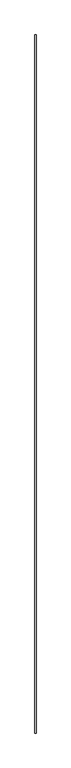
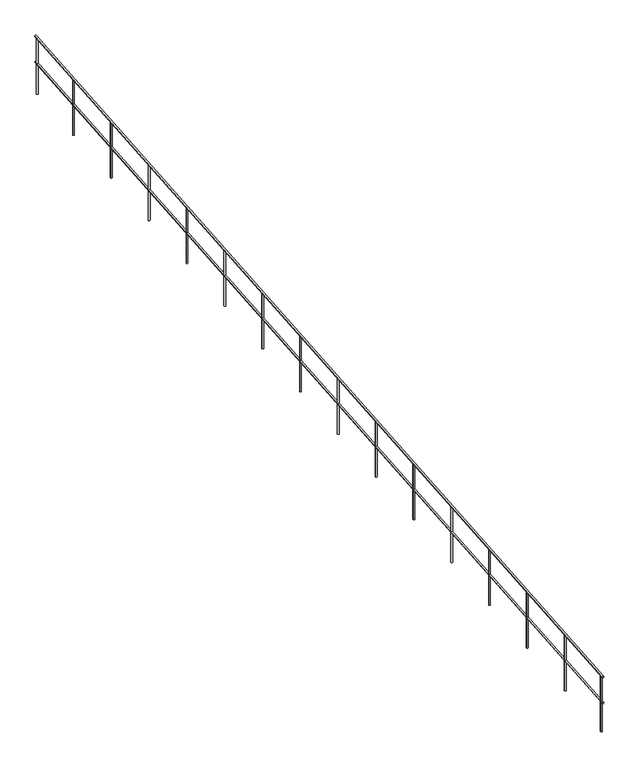
"""IFC4 building model written with IfcOpenShell, lengths in millimetres: railing geometry."""

from ifc_helpers import new_model, si_unit, frame, origin, place, context, project, spatial, ellipse_curve, source, transform, mapped, element, save
from ifc_brep_helpers import plane_surface, cylinder_surface, advanced_brep


def railing_739abddc(model_context):
    return source(origin(), model_context, "Body", "AdvancedBrep", [
        advanced_brep(
        [(-4051.0, 39498.9598199, -615.0519932), (-4081.0, 39498.9598199, -615.0519932), (-4051.0, 57498.9598198, 884.9480068), (-4081.0, 57498.9598198, 884.9480068)],
        [
            (0, 1, ellipse_curve(frame((-4066.0, 39498.9598199, -615.0519932), z_axis=(0.0, -1.0, 0.0), x_axis=(0.0, 0.0, -0.9999999999999999)), 15.0519932, 15.0)),
            (1, 0, ellipse_curve(frame((-4066.0, 39498.9598199, -615.0519932), z_axis=(0.0, -1.0, 0.0), x_axis=(0.0, 0.0, -0.9999999999999999)), 15.0519932, 15.0)),
            (2, 3, ellipse_curve(frame((-4066.0, 57498.9598198, 884.9480068), z_axis=(0.0, 1.0, 0.0), x_axis=(0.0, 0.0, -0.9999999999999999)), 15.0519932, 15.0)),
            (3, 2, ellipse_curve(frame((-4066.0, 57498.9598198, 884.9480068), z_axis=(0.0, 1.0, 0.0), x_axis=(0.0, 0.0, -0.9999999999999999)), 15.0519932, 15.0)),
            (0, 2),
            (3, 1),
        ],
        [
            plane_surface(frame((-4066.0, 39498.9598199, -600.0), z_axis=(0.0, -1.0, 0.0), x_axis=(0.0, 0.0, 1.0))),
            plane_surface(frame((-4066.0, 57498.9598198, 900.0), z_axis=(0.0, 1.0, 0.0), x_axis=(0.0, 0.0, 1.0))),
            cylinder_surface(frame((-4066.0, 39500.2055021, -614.9481864), z_axis=(0.0, -0.9965457582448797, -0.08304547985373997), x_axis=(-1.0, 0.0, 0.0)), 15.0),
        ],
        [
            (0, [[1, 2]]),
            (1, [[3, 4]]),
            (2, [[-1, 5, -4, 6]]),
            (2, [[-2, -6, -3, -5]]),
        ],
    ),
        advanced_brep(
        [(-4051.0, 39498.9598199, -115.0519932), (-4081.0, 39498.9598199, -115.0519932), (-4051.0, 57498.9598198, 1384.9480068), (-4081.0, 57498.9598198, 1384.9480068)],
        [
            (0, 1, ellipse_curve(frame((-4066.0, 39498.9598199, -115.0519932), z_axis=(0.0, -1.0, 0.0), x_axis=(0.0, 0.0, -0.9999999999999999)), 15.0519932, 15.0)),
            (1, 0, ellipse_curve(frame((-4066.0, 39498.9598199, -115.0519932), z_axis=(0.0, -1.0, 0.0), x_axis=(0.0, 0.0, -0.9999999999999999)), 15.0519932, 15.0)),
            (2, 3, ellipse_curve(frame((-4066.0, 57498.9598198, 1384.9480068), z_axis=(0.0, 1.0, 0.0), x_axis=(0.0, 0.0, -0.9999999999999999)), 15.0519932, 15.0)),
            (3, 2, ellipse_curve(frame((-4066.0, 57498.9598198, 1384.9480068), z_axis=(0.0, 1.0, 0.0), x_axis=(0.0, 0.0, -0.9999999999999999)), 15.0519932, 15.0)),
            (0, 2),
            (3, 1),
        ],
        [
            plane_surface(frame((-4066.0, 39498.9598199, -100.0), z_axis=(0.0, -1.0, 0.0), x_axis=(0.0, 0.0, 1.0))),
            plane_surface(frame((-4066.0, 57498.9598198, 1400.0), z_axis=(0.0, 1.0, 0.0), x_axis=(0.0, 0.0, 1.0))),
            cylinder_surface(frame((-4066.0, 39500.2055021, -114.9481864), z_axis=(0.0, -0.9965457582448797, -0.08304547985373997), x_axis=(-1.0, 0.0, 0.0)), 15.0),
        ],
        [
            (0, [[1, 2]]),
            (1, [[3, 4]]),
            (2, [[-1, 5, -4, 6]]),
            (2, [[-2, -6, -3, -5]]),
        ],
    ),
        advanced_brep(
        [(-4081.0, 56298.9598199, 1269.8960136), (-4051.0, 56298.9598199, 1269.8960136), (-4051.0, 56298.9598199, 200.0), (-4081.0, 56298.9598199, 200.0)],
        [
            (0, 1, ellipse_curve(frame((-4066.0, 56298.9598199, 1269.8960136), z_axis=(0.0, 0.083045479853741, -0.9965457582448796), x_axis=(0.0, 0.9965457582448797, 0.08304547985374044)), 15.0519932, 15.0)),
            (1, 2),
            (2, 3, ellipse_curve(frame((-4066.0, 56298.9598199, 200.0), z_axis=(0.0, -0.08304547985373996, 0.9965457582448797), x_axis=(0.0, 0.9965457582448798, 0.08304547985373881)), 15.0519932, 15.0)),
            (3, 0),
            (3, 2, ellipse_curve(frame((-4066.0, 56298.9598199, 200.0), z_axis=(0.0, -0.08304547985373996, 0.9965457582448797), x_axis=(0.0, 0.9965457582448798, 0.08304547985373881)), 15.0519932, 15.0)),
            (1, 0, ellipse_curve(frame((-4066.0, 56298.9598199, 1269.8960136), z_axis=(0.0, 0.083045479853741, -0.9965457582448796), x_axis=(0.0, 0.9965457582448797, 0.08304547985374044)), 15.0519932, 15.0)),
        ],
        [
            cylinder_surface(frame((-4066.0, 56298.9598199, 100.0), z_axis=(0.0, 0.0, 1.0), x_axis=(1.0, 0.0, 0.0)), 15.0),
            plane_surface(frame((-4041.0, 56323.9598199, 1271.9793469), z_axis=(0.0, -0.083045479853741, 0.9965457582448796), x_axis=(-1.0, 0.0, 0.0))),
            plane_surface(frame((-4041.0, 56273.9598199, 197.9166667), z_axis=(0.0, 0.08304547985373996, -0.9965457582448797), x_axis=(-1.0, 0.0, 0.0))),
        ],
        [
            (0, [[1, 2, 3, 4]]),
            (0, [[5, -2, 6, -4]]),
            (1, [[-6, -1]]),
            (2, [[-5, -3]]),
        ],
    ),
        advanced_brep(
        [(-4081.0, 55098.9598199, 1169.8960136), (-4051.0, 55098.9598199, 1169.8960136), (-4051.0, 55098.9598199, 100.0), (-4081.0, 55098.9598199, 100.0)],
        [
            (0, 1, ellipse_curve(frame((-4066.0, 55098.9598199, 1169.8960136), z_axis=(0.0, 0.083045479853741, -0.9965457582448796), x_axis=(0.0, 0.9965457582448797, 0.08304547985374044)), 15.0519932, 15.0)),
            (1, 2),
            (2, 3, ellipse_curve(frame((-4066.0, 55098.9598199, 100.0), z_axis=(0.0, -0.08304547985373996, 0.9965457582448797), x_axis=(0.0, 0.9965457582448798, 0.08304547985373881)), 15.0519932, 15.0)),
            (3, 0),
            (3, 2, ellipse_curve(frame((-4066.0, 55098.9598199, 100.0), z_axis=(0.0, -0.08304547985373996, 0.9965457582448797), x_axis=(0.0, 0.9965457582448798, 0.08304547985373881)), 15.0519932, 15.0)),
            (1, 0, ellipse_curve(frame((-4066.0, 55098.9598199, 1169.8960136), z_axis=(0.0, 0.083045479853741, -0.9965457582448796), x_axis=(0.0, 0.9965457582448797, 0.08304547985374044)), 15.0519932, 15.0)),
        ],
        [
            cylinder_surface(frame((-4066.0, 55098.9598199, 0.0), z_axis=(0.0, 0.0, 1.0), x_axis=(1.0, 0.0, 0.0)), 15.0),
            plane_surface(frame((-4041.0, 55123.9598199, 1171.9793469), z_axis=(0.0, -0.083045479853741, 0.9965457582448796), x_axis=(-1.0, 0.0, 0.0))),
            plane_surface(frame((-4041.0, 55073.9598199, 97.9166667), z_axis=(0.0, 0.08304547985373996, -0.9965457582448797), x_axis=(-1.0, 0.0, 0.0))),
        ],
        [
            (0, [[1, 2, 3, 4]]),
            (0, [[5, -2, 6, -4]]),
            (1, [[-6, -1]]),
            (2, [[-5, -3]]),
        ],
    ),
        advanced_brep(
        [(-4081.0, 53898.9598199, 1069.8960136), (-4051.0, 53898.9598199, 1069.8960136), (-4051.0, 53898.9598199, 0.0), (-4081.0, 53898.9598199, 0.0)],
        [
            (0, 1, ellipse_curve(frame((-4066.0, 53898.9598199, 1069.8960136), z_axis=(0.0, 0.083045479853741, -0.9965457582448796), x_axis=(0.0, 0.9965457582448797, 0.08304547985374044)), 15.0519932, 15.0)),
            (1, 2),
            (2, 3, ellipse_curve(frame((-4066.0, 53898.9598199, 0.0), z_axis=(0.0, -0.08304547985373996, 0.9965457582448797), x_axis=(0.0, 0.9965457582448798, 0.08304547985373881)), 15.0519932, 15.0)),
            (3, 0),
            (3, 2, ellipse_curve(frame((-4066.0, 53898.9598199, 0.0), z_axis=(0.0, -0.08304547985373996, 0.9965457582448797), x_axis=(0.0, 0.9965457582448798, 0.08304547985373881)), 15.0519932, 15.0)),
            (1, 0, ellipse_curve(frame((-4066.0, 53898.9598199, 1069.8960136), z_axis=(0.0, 0.083045479853741, -0.9965457582448796), x_axis=(0.0, 0.9965457582448797, 0.08304547985374044)), 15.0519932, 15.0)),
        ],
        [
            cylinder_surface(frame((-4066.0, 53898.9598199, -100.0), z_axis=(0.0, 0.0, 1.0), x_axis=(1.0, 0.0, 0.0)), 15.0),
            plane_surface(frame((-4041.0, 53923.9598199, 1071.9793469), z_axis=(0.0, -0.083045479853741, 0.9965457582448796), x_axis=(-1.0, 0.0, 0.0))),
            plane_surface(frame((-4041.0, 53873.9598199, -2.0833333), z_axis=(0.0, 0.08304547985373996, -0.9965457582448797), x_axis=(-1.0, 0.0, 0.0))),
        ],
        [
            (0, [[1, 2, 3, 4]]),
            (0, [[5, -2, 6, -4]]),
            (1, [[-6, -1]]),
            (2, [[-5, -3]]),
        ],
    ),
        advanced_brep(
        [(-4081.0, 52698.9598199, 969.8960136), (-4051.0, 52698.9598199, 969.8960136), (-4051.0, 52698.9598199, -100.0), (-4081.0, 52698.9598199, -100.0)],
        [
            (0, 1, ellipse_curve(frame((-4066.0, 52698.9598199, 969.8960136), z_axis=(0.0, 0.083045479853741, -0.9965457582448796), x_axis=(0.0, 0.9965457582448797, 0.08304547985374044)), 15.0519932, 15.0)),
            (1, 2),
            (2, 3, ellipse_curve(frame((-4066.0, 52698.9598199, -100.0), z_axis=(0.0, -0.08304547985373996, 0.9965457582448797), x_axis=(0.0, 0.9965457582448798, 0.08304547985373881)), 15.0519932, 15.0)),
            (3, 0),
            (3, 2, ellipse_curve(frame((-4066.0, 52698.9598199, -100.0), z_axis=(0.0, -0.08304547985373996, 0.9965457582448797), x_axis=(0.0, 0.9965457582448798, 0.08304547985373881)), 15.0519932, 15.0)),
            (1, 0, ellipse_curve(frame((-4066.0, 52698.9598199, 969.8960136), z_axis=(0.0, 0.083045479853741, -0.9965457582448796), x_axis=(0.0, 0.9965457582448797, 0.08304547985374044)), 15.0519932, 15.0)),
        ],
        [
            cylinder_surface(frame((-4066.0, 52698.9598199, -200.0), z_axis=(0.0, 0.0, 1.0), x_axis=(1.0, 0.0, 0.0)), 15.0),
            plane_surface(frame((-4041.0, 52723.9598199, 971.9793469), z_axis=(0.0, -0.083045479853741, 0.9965457582448796), x_axis=(-1.0, 0.0, 0.0))),
            plane_surface(frame((-4041.0, 52673.9598199, -102.0833333), z_axis=(0.0, 0.08304547985373996, -0.9965457582448797), x_axis=(-1.0, 0.0, 0.0))),
        ],
        [
            (0, [[1, 2, 3, 4]]),
            (0, [[5, -2, 6, -4]]),
            (1, [[-6, -1]]),
            (2, [[-5, -3]]),
        ],
    ),
        advanced_brep(
        [(-4081.0, 51498.9598199, 869.8960136), (-4051.0, 51498.9598199, 869.8960136), (-4051.0, 51498.9598199, -200.0), (-4081.0, 51498.9598199, -200.0)],
        [
            (0, 1, ellipse_curve(frame((-4066.0, 51498.9598199, 869.8960136), z_axis=(0.0, 0.083045479853741, -0.9965457582448796), x_axis=(0.0, 0.9965457582448797, 0.08304547985374044)), 15.0519932, 15.0)),
            (1, 2),
            (2, 3, ellipse_curve(frame((-4066.0, 51498.9598199, -200.0), z_axis=(0.0, -0.08304547985373996, 0.9965457582448797), x_axis=(0.0, 0.9965457582448798, 0.08304547985373881)), 15.0519932, 15.0)),
            (3, 0),
            (3, 2, ellipse_curve(frame((-4066.0, 51498.9598199, -200.0), z_axis=(0.0, -0.08304547985373996, 0.9965457582448797), x_axis=(0.0, 0.9965457582448798, 0.08304547985373881)), 15.0519932, 15.0)),
            (1, 0, ellipse_curve(frame((-4066.0, 51498.9598199, 869.8960136), z_axis=(0.0, 0.083045479853741, -0.9965457582448796), x_axis=(0.0, 0.9965457582448797, 0.08304547985374044)), 15.0519932, 15.0)),
        ],
        [
            cylinder_surface(frame((-4066.0, 51498.9598199, -300.0), z_axis=(0.0, 0.0, 1.0), x_axis=(1.0, 0.0, 0.0)), 15.0),
            plane_surface(frame((-4041.0, 51523.9598199, 871.9793469), z_axis=(0.0, -0.083045479853741, 0.9965457582448796), x_axis=(-1.0, 0.0, 0.0))),
            plane_surface(frame((-4041.0, 51473.9598199, -202.0833333), z_axis=(0.0, 0.08304547985373996, -0.9965457582448797), x_axis=(-1.0, 0.0, 0.0))),
        ],
        [
            (0, [[1, 2, 3, 4]]),
            (0, [[5, -2, 6, -4]]),
            (1, [[-6, -1]]),
            (2, [[-5, -3]]),
        ],
    ),
        advanced_brep(
        [(-4081.0, 50298.9598199, 769.8960136), (-4051.0, 50298.9598199, 769.8960136), (-4051.0, 50298.9598199, -300.0), (-4081.0, 50298.9598199, -300.0)],
        [
            (0, 1, ellipse_curve(frame((-4066.0, 50298.9598199, 769.8960136), z_axis=(0.0, 0.083045479853741, -0.9965457582448796), x_axis=(0.0, 0.9965457582448797, 0.08304547985374044)), 15.0519932, 15.0)),
            (1, 2),
            (2, 3, ellipse_curve(frame((-4066.0, 50298.9598199, -300.0), z_axis=(0.0, -0.08304547985373996, 0.9965457582448797), x_axis=(0.0, 0.9965457582448798, 0.08304547985373881)), 15.0519932, 15.0)),
            (3, 0),
            (3, 2, ellipse_curve(frame((-4066.0, 50298.9598199, -300.0), z_axis=(0.0, -0.08304547985373996, 0.9965457582448797), x_axis=(0.0, 0.9965457582448798, 0.08304547985373881)), 15.0519932, 15.0)),
            (1, 0, ellipse_curve(frame((-4066.0, 50298.9598199, 769.8960136), z_axis=(0.0, 0.083045479853741, -0.9965457582448796), x_axis=(0.0, 0.9965457582448797, 0.08304547985374044)), 15.0519932, 15.0)),
        ],
        [
            cylinder_surface(frame((-4066.0, 50298.9598199, -400.0), z_axis=(0.0, 0.0, 1.0), x_axis=(1.0, 0.0, 0.0)), 15.0),
            plane_surface(frame((-4041.0, 50323.9598199, 771.9793469), z_axis=(0.0, -0.083045479853741, 0.9965457582448796), x_axis=(-1.0, 0.0, 0.0))),
            plane_surface(frame((-4041.0, 50273.9598199, -302.0833333), z_axis=(0.0, 0.08304547985373996, -0.9965457582448797), x_axis=(-1.0, 0.0, 0.0))),
        ],
        [
            (0, [[1, 2, 3, 4]]),
            (0, [[5, -2, 6, -4]]),
            (1, [[-6, -1]]),
            (2, [[-5, -3]]),
        ],
    ),
        advanced_brep(
        [(-4081.0, 49098.9598199, 669.8960136), (-4051.0, 49098.9598199, 669.8960136), (-4051.0, 49098.9598199, -400.0), (-4081.0, 49098.9598199, -400.0)],
        [
            (0, 1, ellipse_curve(frame((-4066.0, 49098.9598199, 669.8960136), z_axis=(0.0, 0.083045479853741, -0.9965457582448796), x_axis=(0.0, 0.9965457582448797, 0.08304547985374044)), 15.0519932, 15.0)),
            (1, 2),
            (2, 3, ellipse_curve(frame((-4066.0, 49098.9598199, -400.0), z_axis=(0.0, -0.08304547985373996, 0.9965457582448797), x_axis=(0.0, 0.9965457582448798, 0.08304547985373881)), 15.0519932, 15.0)),
            (3, 0),
            (3, 2, ellipse_curve(frame((-4066.0, 49098.9598199, -400.0), z_axis=(0.0, -0.08304547985373996, 0.9965457582448797), x_axis=(0.0, 0.9965457582448798, 0.08304547985373881)), 15.0519932, 15.0)),
            (1, 0, ellipse_curve(frame((-4066.0, 49098.9598199, 669.8960136), z_axis=(0.0, 0.083045479853741, -0.9965457582448796), x_axis=(0.0, 0.9965457582448797, 0.08304547985374044)), 15.0519932, 15.0)),
        ],
        [
            cylinder_surface(frame((-4066.0, 49098.9598199, -500.0), z_axis=(0.0, 0.0, 1.0), x_axis=(1.0, 0.0, 0.0)), 15.0),
            plane_surface(frame((-4041.0, 49123.9598199, 671.9793469), z_axis=(0.0, -0.083045479853741, 0.9965457582448796), x_axis=(-1.0, 0.0, 0.0))),
            plane_surface(frame((-4041.0, 49073.9598199, -402.0833333), z_axis=(0.0, 0.08304547985373996, -0.9965457582448797), x_axis=(-1.0, 0.0, 0.0))),
        ],
        [
            (0, [[1, 2, 3, 4]]),
            (0, [[5, -2, 6, -4]]),
            (1, [[-6, -1]]),
            (2, [[-5, -3]]),
        ],
    ),
        advanced_brep(
        [(-4081.0, 47898.9598199, 569.8960136), (-4051.0, 47898.9598199, 569.8960136), (-4051.0, 47898.9598199, -500.0), (-4081.0, 47898.9598199, -500.0)],
        [
            (0, 1, ellipse_curve(frame((-4066.0, 47898.9598199, 569.8960136), z_axis=(0.0, 0.083045479853741, -0.9965457582448796), x_axis=(0.0, 0.9965457582448797, 0.08304547985374044)), 15.0519932, 15.0)),
            (1, 2),
            (2, 3, ellipse_curve(frame((-4066.0, 47898.9598199, -500.0), z_axis=(0.0, -0.08304547985373996, 0.9965457582448797), x_axis=(0.0, 0.9965457582448798, 0.08304547985373881)), 15.0519932, 15.0)),
            (3, 0),
            (3, 2, ellipse_curve(frame((-4066.0, 47898.9598199, -500.0), z_axis=(0.0, -0.08304547985373996, 0.9965457582448797), x_axis=(0.0, 0.9965457582448798, 0.08304547985373881)), 15.0519932, 15.0)),
            (1, 0, ellipse_curve(frame((-4066.0, 47898.9598199, 569.8960136), z_axis=(0.0, 0.083045479853741, -0.9965457582448796), x_axis=(0.0, 0.9965457582448797, 0.08304547985374044)), 15.0519932, 15.0)),
        ],
        [
            cylinder_surface(frame((-4066.0, 47898.9598199, -600.0), z_axis=(0.0, 0.0, 1.0), x_axis=(1.0, 0.0, 0.0)), 15.0),
            plane_surface(frame((-4041.0, 47923.9598199, 571.9793469), z_axis=(0.0, -0.083045479853741, 0.9965457582448796), x_axis=(-1.0, 0.0, 0.0))),
            plane_surface(frame((-4041.0, 47873.9598199, -502.0833333), z_axis=(0.0, 0.08304547985373996, -0.9965457582448797), x_axis=(-1.0, 0.0, 0.0))),
        ],
        [
            (0, [[1, 2, 3, 4]]),
            (0, [[5, -2, 6, -4]]),
            (1, [[-6, -1]]),
            (2, [[-5, -3]]),
        ],
    ),
        advanced_brep(
        [(-4081.0, 46698.9598199, 469.8960136), (-4051.0, 46698.9598199, 469.8960136), (-4051.0, 46698.9598199, -600.0), (-4081.0, 46698.9598199, -600.0)],
        [
            (0, 1, ellipse_curve(frame((-4066.0, 46698.9598199, 469.8960136), z_axis=(0.0, 0.083045479853741, -0.9965457582448796), x_axis=(0.0, 0.9965457582448797, 0.08304547985374044)), 15.0519932, 15.0)),
            (1, 2),
            (2, 3, ellipse_curve(frame((-4066.0, 46698.9598199, -600.0), z_axis=(0.0, -0.08304547985373996, 0.9965457582448797), x_axis=(0.0, 0.9965457582448798, 0.08304547985373881)), 15.0519932, 15.0)),
            (3, 0),
            (3, 2, ellipse_curve(frame((-4066.0, 46698.9598199, -600.0), z_axis=(0.0, -0.08304547985373996, 0.9965457582448797), x_axis=(0.0, 0.9965457582448798, 0.08304547985373881)), 15.0519932, 15.0)),
            (1, 0, ellipse_curve(frame((-4066.0, 46698.9598199, 469.8960136), z_axis=(0.0, 0.083045479853741, -0.9965457582448796), x_axis=(0.0, 0.9965457582448797, 0.08304547985374044)), 15.0519932, 15.0)),
        ],
        [
            cylinder_surface(frame((-4066.0, 46698.9598199, -700.0), z_axis=(0.0, 0.0, 1.0), x_axis=(1.0, 0.0, 0.0)), 15.0),
            plane_surface(frame((-4041.0, 46723.9598199, 471.9793469), z_axis=(0.0, -0.083045479853741, 0.9965457582448796), x_axis=(-1.0, 0.0, 0.0))),
            plane_surface(frame((-4041.0, 46673.9598199, -602.0833333), z_axis=(0.0, 0.08304547985373996, -0.9965457582448797), x_axis=(-1.0, 0.0, 0.0))),
        ],
        [
            (0, [[1, 2, 3, 4]]),
            (0, [[5, -2, 6, -4]]),
            (1, [[-6, -1]]),
            (2, [[-5, -3]]),
        ],
    ),
        advanced_brep(
        [(-4081.0, 45498.9598199, 369.8960136), (-4051.0, 45498.9598199, 369.8960136), (-4051.0, 45498.9598199, -700.0), (-4081.0, 45498.9598199, -700.0)],
        [
            (0, 1, ellipse_curve(frame((-4066.0, 45498.9598199, 369.8960136), z_axis=(0.0, 0.083045479853741, -0.9965457582448796), x_axis=(0.0, 0.9965457582448797, 0.08304547985374044)), 15.0519932, 15.0)),
            (1, 2),
            (2, 3, ellipse_curve(frame((-4066.0, 45498.9598199, -700.0), z_axis=(0.0, -0.08304547985373996, 0.9965457582448797), x_axis=(0.0, 0.9965457582448798, 0.08304547985373881)), 15.0519932, 15.0)),
            (3, 0),
            (3, 2, ellipse_curve(frame((-4066.0, 45498.9598199, -700.0), z_axis=(0.0, -0.08304547985373996, 0.9965457582448797), x_axis=(0.0, 0.9965457582448798, 0.08304547985373881)), 15.0519932, 15.0)),
            (1, 0, ellipse_curve(frame((-4066.0, 45498.9598199, 369.8960136), z_axis=(0.0, 0.083045479853741, -0.9965457582448796), x_axis=(0.0, 0.9965457582448797, 0.08304547985374044)), 15.0519932, 15.0)),
        ],
        [
            cylinder_surface(frame((-4066.0, 45498.9598199, -800.0), z_axis=(0.0, 0.0, 1.0), x_axis=(1.0, 0.0, 0.0)), 15.0),
            plane_surface(frame((-4041.0, 45523.9598199, 371.9793469), z_axis=(0.0, -0.083045479853741, 0.9965457582448796), x_axis=(-1.0, 0.0, 0.0))),
            plane_surface(frame((-4041.0, 45473.9598199, -702.0833333), z_axis=(0.0, 0.08304547985373996, -0.9965457582448797), x_axis=(-1.0, 0.0, 0.0))),
        ],
        [
            (0, [[1, 2, 3, 4]]),
            (0, [[5, -2, 6, -4]]),
            (1, [[-6, -1]]),
            (2, [[-5, -3]]),
        ],
    ),
        advanced_brep(
        [(-4081.0, 44298.9598199, 269.8960136), (-4051.0, 44298.9598199, 269.8960136), (-4051.0, 44298.9598199, -800.0), (-4081.0, 44298.9598199, -800.0)],
        [
            (0, 1, ellipse_curve(frame((-4066.0, 44298.9598199, 269.8960136), z_axis=(0.0, 0.083045479853741, -0.9965457582448796), x_axis=(0.0, 0.9965457582448797, 0.08304547985374044)), 15.0519932, 15.0)),
            (1, 2),
            (2, 3, ellipse_curve(frame((-4066.0, 44298.9598199, -800.0), z_axis=(0.0, -0.08304547985373996, 0.9965457582448797), x_axis=(0.0, 0.9965457582448798, 0.08304547985373881)), 15.0519932, 15.0)),
            (3, 0),
            (3, 2, ellipse_curve(frame((-4066.0, 44298.9598199, -800.0), z_axis=(0.0, -0.08304547985373996, 0.9965457582448797), x_axis=(0.0, 0.9965457582448798, 0.08304547985373881)), 15.0519932, 15.0)),
            (1, 0, ellipse_curve(frame((-4066.0, 44298.9598199, 269.8960136), z_axis=(0.0, 0.083045479853741, -0.9965457582448796), x_axis=(0.0, 0.9965457582448797, 0.08304547985374044)), 15.0519932, 15.0)),
        ],
        [
            cylinder_surface(frame((-4066.0, 44298.9598199, -900.0), z_axis=(0.0, 0.0, 1.0), x_axis=(1.0, 0.0, 0.0)), 15.0),
            plane_surface(frame((-4041.0, 44323.9598199, 271.9793469), z_axis=(0.0, -0.083045479853741, 0.9965457582448796), x_axis=(-1.0, 0.0, 0.0))),
            plane_surface(frame((-4041.0, 44273.9598199, -802.0833333), z_axis=(0.0, 0.08304547985373996, -0.9965457582448797), x_axis=(-1.0, 0.0, 0.0))),
        ],
        [
            (0, [[1, 2, 3, 4]]),
            (0, [[5, -2, 6, -4]]),
            (1, [[-6, -1]]),
            (2, [[-5, -3]]),
        ],
    ),
        advanced_brep(
        [(-4081.0, 43098.9598199, 169.8960136), (-4051.0, 43098.9598199, 169.8960136), (-4051.0, 43098.9598199, -900.0), (-4081.0, 43098.9598199, -900.0)],
        [
            (0, 1, ellipse_curve(frame((-4066.0, 43098.9598199, 169.8960136), z_axis=(0.0, 0.083045479853741, -0.9965457582448796), x_axis=(0.0, 0.9965457582448797, 0.08304547985374044)), 15.0519932, 15.0)),
            (1, 2),
            (2, 3, ellipse_curve(frame((-4066.0, 43098.9598199, -900.0), z_axis=(0.0, -0.08304547985373996, 0.9965457582448797), x_axis=(0.0, 0.9965457582448798, 0.08304547985373881)), 15.0519932, 15.0)),
            (3, 0),
            (3, 2, ellipse_curve(frame((-4066.0, 43098.9598199, -900.0), z_axis=(0.0, -0.08304547985373996, 0.9965457582448797), x_axis=(0.0, 0.9965457582448798, 0.08304547985373881)), 15.0519932, 15.0)),
            (1, 0, ellipse_curve(frame((-4066.0, 43098.9598199, 169.8960136), z_axis=(0.0, 0.083045479853741, -0.9965457582448796), x_axis=(0.0, 0.9965457582448797, 0.08304547985374044)), 15.0519932, 15.0)),
        ],
        [
            cylinder_surface(frame((-4066.0, 43098.9598199, -1000.0), z_axis=(0.0, 0.0, 1.0), x_axis=(1.0, 0.0, 0.0)), 15.0),
            plane_surface(frame((-4041.0, 43123.9598199, 171.9793469), z_axis=(0.0, -0.083045479853741, 0.9965457582448796), x_axis=(-1.0, 0.0, 0.0))),
            plane_surface(frame((-4041.0, 43073.9598199, -902.0833333), z_axis=(0.0, 0.08304547985373996, -0.9965457582448797), x_axis=(-1.0, 0.0, 0.0))),
        ],
        [
            (0, [[1, 2, 3, 4]]),
            (0, [[5, -2, 6, -4]]),
            (1, [[-6, -1]]),
            (2, [[-5, -3]]),
        ],
    ),
        advanced_brep(
        [(-4081.0, 41898.9598199, 69.8960136), (-4051.0, 41898.9598199, 69.8960136), (-4051.0, 41898.9598199, -1000.0), (-4081.0, 41898.9598199, -1000.0)],
        [
            (0, 1, ellipse_curve(frame((-4066.0, 41898.9598199, 69.8960136), z_axis=(0.0, 0.083045479853741, -0.9965457582448796), x_axis=(0.0, 0.9965457582448797, 0.08304547985374044)), 15.0519932, 15.0)),
            (1, 2),
            (2, 3, ellipse_curve(frame((-4066.0, 41898.9598199, -1000.0), z_axis=(0.0, -0.08304547985373996, 0.9965457582448797), x_axis=(0.0, 0.9965457582448798, 0.08304547985373881)), 15.0519932, 15.0)),
            (3, 0),
            (3, 2, ellipse_curve(frame((-4066.0, 41898.9598199, -1000.0), z_axis=(0.0, -0.08304547985373996, 0.9965457582448797), x_axis=(0.0, 0.9965457582448798, 0.08304547985373881)), 15.0519932, 15.0)),
            (1, 0, ellipse_curve(frame((-4066.0, 41898.9598199, 69.8960136), z_axis=(0.0, 0.083045479853741, -0.9965457582448796), x_axis=(0.0, 0.9965457582448797, 0.08304547985374044)), 15.0519932, 15.0)),
        ],
        [
            cylinder_surface(frame((-4066.0, 41898.9598199, -1100.0), z_axis=(0.0, 0.0, 1.0), x_axis=(1.0, 0.0, 0.0)), 15.0),
            plane_surface(frame((-4041.0, 41923.9598199, 71.9793469), z_axis=(0.0, -0.083045479853741, 0.9965457582448796), x_axis=(-1.0, 0.0, 0.0))),
            plane_surface(frame((-4041.0, 41873.9598199, -1002.0833333), z_axis=(0.0, 0.08304547985373996, -0.9965457582448797), x_axis=(-1.0, 0.0, 0.0))),
        ],
        [
            (0, [[1, 2, 3, 4]]),
            (0, [[5, -2, 6, -4]]),
            (1, [[-6, -1]]),
            (2, [[-5, -3]]),
        ],
    ),
        advanced_brep(
        [(-4081.0, 40698.9598199, -30.1039864), (-4051.0, 40698.9598199, -30.1039864), (-4051.0, 40698.9598199, -1100.0), (-4081.0, 40698.9598199, -1100.0)],
        [
            (0, 1, ellipse_curve(frame((-4066.0, 40698.9598199, -30.1039864), z_axis=(0.0, 0.083045479853741, -0.9965457582448796), x_axis=(0.0, 0.9965457582448797, 0.08304547985374044)), 15.0519932, 15.0)),
            (1, 2),
            (2, 3, ellipse_curve(frame((-4066.0, 40698.9598199, -1100.0), z_axis=(0.0, -0.08304547985373996, 0.9965457582448797), x_axis=(0.0, 0.9965457582448798, 0.08304547985373881)), 15.0519932, 15.0)),
            (3, 0),
            (3, 2, ellipse_curve(frame((-4066.0, 40698.9598199, -1100.0), z_axis=(0.0, -0.08304547985373996, 0.9965457582448797), x_axis=(0.0, 0.9965457582448798, 0.08304547985373881)), 15.0519932, 15.0)),
            (1, 0, ellipse_curve(frame((-4066.0, 40698.9598199, -30.1039864), z_axis=(0.0, 0.083045479853741, -0.9965457582448796), x_axis=(0.0, 0.9965457582448797, 0.08304547985374044)), 15.0519932, 15.0)),
        ],
        [
            cylinder_surface(frame((-4066.0, 40698.9598199, -1200.0), z_axis=(0.0, 0.0, 1.0), x_axis=(1.0, 0.0, 0.0)), 15.0),
            plane_surface(frame((-4041.0, 40723.9598199, -28.0206531), z_axis=(0.0, -0.083045479853741, 0.9965457582448796), x_axis=(-1.0, 0.0, 0.0))),
            plane_surface(frame((-4041.0, 40673.9598199, -1102.0833333), z_axis=(0.0, 0.08304547985373996, -0.9965457582448797), x_axis=(-1.0, 0.0, 0.0))),
        ],
        [
            (0, [[1, 2, 3, 4]]),
            (0, [[5, -2, 6, -4]]),
            (1, [[-6, -1]]),
            (2, [[-5, -3]]),
        ],
    ),
        advanced_brep(
        [(-4081.0, 57448.9598198, 1365.7293469), (-4051.0, 57448.9598198, 1365.7293469), (-4051.0, 57448.9598198, 295.8333333), (-4081.0, 57448.9598198, 295.8333333)],
        [
            (0, 1, ellipse_curve(frame((-4066.0, 57448.9598198, 1365.7293469), z_axis=(0.0, 0.083045479853741, -0.9965457582448796), x_axis=(0.0, 0.9965457582448797, 0.08304547985374044)), 15.0519932, 15.0)),
            (1, 2),
            (2, 3, ellipse_curve(frame((-4066.0, 57448.9598198, 295.8333333), z_axis=(0.0, -0.08304547985373996, 0.9965457582448797), x_axis=(0.0, 0.9965457582448798, 0.08304547985373881)), 15.0519932, 15.0)),
            (3, 0),
            (3, 2, ellipse_curve(frame((-4066.0, 57448.9598198, 295.8333333), z_axis=(0.0, -0.08304547985373996, 0.9965457582448797), x_axis=(0.0, 0.9965457582448798, 0.08304547985373881)), 15.0519932, 15.0)),
            (1, 0, ellipse_curve(frame((-4066.0, 57448.9598198, 1365.7293469), z_axis=(0.0, 0.083045479853741, -0.9965457582448796), x_axis=(0.0, 0.9965457582448797, 0.08304547985374044)), 15.0519932, 15.0)),
        ],
        [
            cylinder_surface(frame((-4066.0, 57448.9598198, 195.8333333), z_axis=(0.0, 0.0, 1.0), x_axis=(1.0, 0.0, 0.0)), 15.0),
            plane_surface(frame((-4041.0, 57473.9598198, 1367.8126802), z_axis=(0.0, -0.083045479853741, 0.9965457582448796), x_axis=(-1.0, 0.0, 0.0))),
            plane_surface(frame((-4041.0, 57423.9598198, 293.75), z_axis=(0.0, 0.08304547985373996, -0.9965457582448797), x_axis=(-1.0, 0.0, 0.0))),
        ],
        [
            (0, [[1, 2, 3, 4]]),
            (0, [[5, -2, 6, -4]]),
            (1, [[-6, -1]]),
            (2, [[-5, -3]]),
        ],
    ),
        advanced_brep(
        [(-4081.0, 39548.9598199, -125.9373198), (-4051.0, 39548.9598199, -125.9373198), (-4051.0, 39548.9598199, -1195.8333333), (-4081.0, 39548.9598199, -1195.8333333)],
        [
            (0, 1, ellipse_curve(frame((-4066.0, 39548.9598199, -125.9373198), z_axis=(0.0, 0.083045479853741, -0.9965457582448796), x_axis=(0.0, 0.9965457582448797, 0.08304547985374044)), 15.0519932, 15.0)),
            (1, 2),
            (2, 3, ellipse_curve(frame((-4066.0, 39548.9598199, -1195.8333333), z_axis=(0.0, -0.08304547985373996, 0.9965457582448797), x_axis=(0.0, 0.9965457582448798, 0.08304547985373881)), 15.0519932, 15.0)),
            (3, 0),
            (3, 2, ellipse_curve(frame((-4066.0, 39548.9598199, -1195.8333333), z_axis=(0.0, -0.08304547985373996, 0.9965457582448797), x_axis=(0.0, 0.9965457582448798, 0.08304547985373881)), 15.0519932, 15.0)),
            (1, 0, ellipse_curve(frame((-4066.0, 39548.9598199, -125.9373198), z_axis=(0.0, 0.083045479853741, -0.9965457582448796), x_axis=(0.0, 0.9965457582448797, 0.08304547985374044)), 15.0519932, 15.0)),
        ],
        [
            cylinder_surface(frame((-4066.0, 39548.9598199, -1295.8333333), z_axis=(0.0, 0.0, 1.0), x_axis=(1.0, 0.0, 0.0)), 15.0),
            plane_surface(frame((-4041.0, 39573.9598199, -123.8539864), z_axis=(0.0, -0.083045479853741, 0.9965457582448796), x_axis=(-1.0, 0.0, 0.0))),
            plane_surface(frame((-4041.0, 39523.9598199, -1197.9166667), z_axis=(0.0, 0.08304547985373996, -0.9965457582448797), x_axis=(-1.0, 0.0, 0.0))),
        ],
        [
            (0, [[1, 2, 3, 4]]),
            (0, [[5, -2, 6, -4]]),
            (1, [[-6, -1]]),
            (2, [[-5, -3]]),
        ],
    ),
    ])


if __name__ == "__main__":
    model = new_model("IFC4")
    model_context = context("Model", 3, world=origin())
    ifc_project = project(units=[si_unit("LENGTHUNIT", "METRE", prefix="MILLI")], contexts=[model_context])
    site = spatial("IfcSite", under=ifc_project)
    building = spatial("IfcBuilding", under=site)
    placement = place(None, origin())
    railing_shape = railing_739abddc(model_context)
    element("IfcRailing", 1, at=placement, inside=building, context=model_context, shape_type="MappedRepresentation", body=[
        mapped(railing_shape, transform((0.0, 0.0, 0.0), x_axis=(1.0, 0.0, 0.0), y_axis=(0.0, 1.0, 0.0), z_axis=(0.0, 0.0, 1.0))),
    ])
    save(model, "model.ifc")
